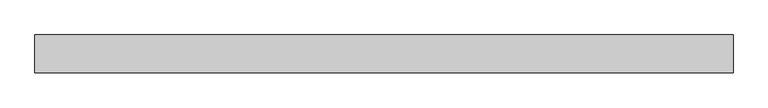
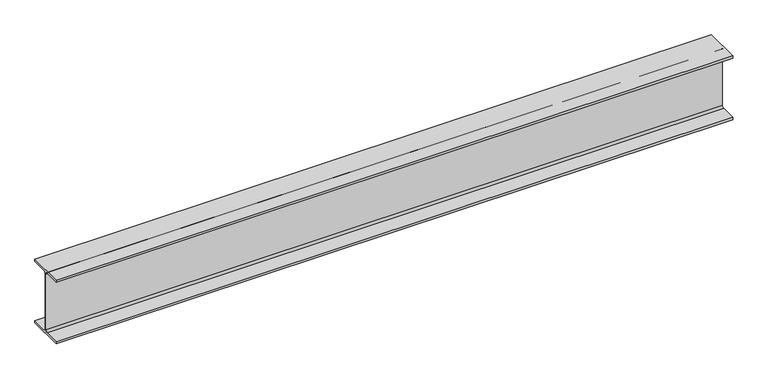
"""IFC4 building model written with IfcOpenShell, lengths in millimetres: beam geometry, Old_Steel Beam_H-KSD3502 : H_SB_ASB_H-200×200x8x12."""

from ifc_helpers import new_model, si_unit, point, frame, frame_2d, origin, place, context, project, spatial, polyline, circle_curve, trimmed, segment, composite_curve, outline, extrude, source, transform, mapped, element, save


def beam_8ff7785c(model_context):
    return source(origin(), model_context, "Body", "SweptSolid", [
        extrude(outline(composite_curve([segment(polyline([(82.5, -141.5), (82.5, -151.7), (-82.5, -151.7), (-82.5, -141.5), (-11.9, -141.5)]), True, "CONTINUOUS"), segment(trimmed(circle_curve(frame_2d((-11.9, -132.6)), 8.9), [point((-11.9, -141.5))], [point((-3.0, -132.6))], True, "CARTESIAN"), True, "CONTINUOUS"), segment(polyline([(-3.0, -132.6), (-3.0, 132.6)]), True, "CONTINUOUS"), segment(trimmed(circle_curve(frame_2d((-11.9, 132.6)), 8.9), [point((-3.0, 132.6))], [point((-11.9, 141.5))], True, "CARTESIAN"), True, "CONTINUOUS"), segment(polyline([(-11.9, 141.5), (-82.5, 141.5), (-82.5, 151.7), (82.5, 151.7), (82.5, 141.5), (11.9, 141.5)]), True, "CONTINUOUS"), segment(trimmed(circle_curve(frame_2d((11.9, 132.6)), 8.9), [point((11.9, 141.5))], [point((3.0, 132.6))], True, "CARTESIAN"), True, "CONTINUOUS"), segment(polyline([(3.0, 132.6), (3.0, -132.6)]), True, "CONTINUOUS"), segment(trimmed(circle_curve(frame_2d((11.9, -132.6)), 8.9), [point((3.0, -132.6))], [point((11.9, -141.5))], True, "CARTESIAN"), True, "CONTINUOUS"), segment(polyline([(11.9, -141.5), (82.5, -141.5)]), True, "CONTINUOUS")], self_intersect=False)), frame((-1343.7619501, 0.0, 0.0), z_axis=(1.0, 0.0, 0.0), x_axis=(0.0, 1.0, 0.0)), (0.0, 0.0, 1.0), 3051.2886648),
    ])


if __name__ == "__main__":
    model = new_model("IFC4")
    model_context = context("Model", 3, world=origin())
    ifc_project = project(units=[si_unit("LENGTHUNIT", "METRE", prefix="MILLI")], contexts=[model_context])
    site = spatial("IfcSite", under=ifc_project)
    building = spatial("IfcBuilding", under=site)
    placement = place(None, origin())
    beam_shape = beam_8ff7785c(model_context)
    element("IfcBeam", 1, ObjectType="Old_Steel Beam_H-KSD3502 : H_SB_ASB_H-200×200x8x12", at=placement, inside=building, context=model_context, shape_type="MappedRepresentation", body=[
        mapped(beam_shape, transform((0.0, 0.0, 0.0), x_axis=(1.0, 0.0, 0.0), y_axis=(0.0, 1.0, 0.0), z_axis=(0.0, 0.0, 1.0))),
    ])
    save(model, "model.ifc")

# Revit data of these elements
# Type "Old_Steel Beam_H-KSD3502 : H_SB_ASB_H-200×200x8x12"
#   Width = 20.0 cm
#   Web Thickness = 0.8 cm
#   Web Fillet = 1.3 cm
#   Warping Constant = 141376.0 cm⁶
#   Torsional Moment of Inertia = 26.2485 cm⁴
#   Torsional Modulus = 1.0 cm³
#   Section Area = 63.53 cm²
#   Plastic Modulus weak axis = 244.0 cm³
#   Plastic Modulus strong axis = 525.0 cm³
#   Perimeter = 1.16 m²/m
#   Nominal Weight = 49.90 kgf/m
#   Moment of Inertia weak axis = 1600.00 cm⁴
#   Moment of Inertia strong axis = 4720.00 cm⁴
#   Height = 20.0 cm
#   Flange Thickness = 1.2 cm
#   Elastic Modulus weak axis = 160.0 cm³
#   Elastic Modulus strong axis = 472.0 cm³
#   Centroid Vertical = 10.0 cm
#   Centroid Horizontal = 10.0 cm
#   Length [instance default] = 1.5240 m
#   Structural Material [instance default] = Steel, 45-345
#   Assembly Code = ""
# Element 1 (IfcBeam, "Old_Steel Beam_H-KSD3502 : H_SB_ASB_H-200×200x8x12")
#   Structural Material = none
# Materials
#   "Steel, 45-345": class "Metal", colour RGB 189 187 185, transparency 0, Description = "Steel 345 MPa", Cost = 0
